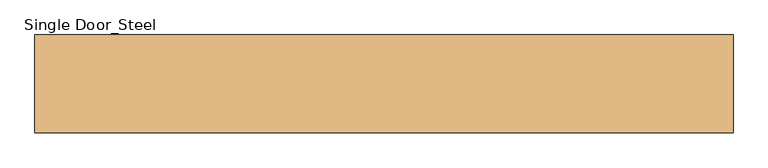
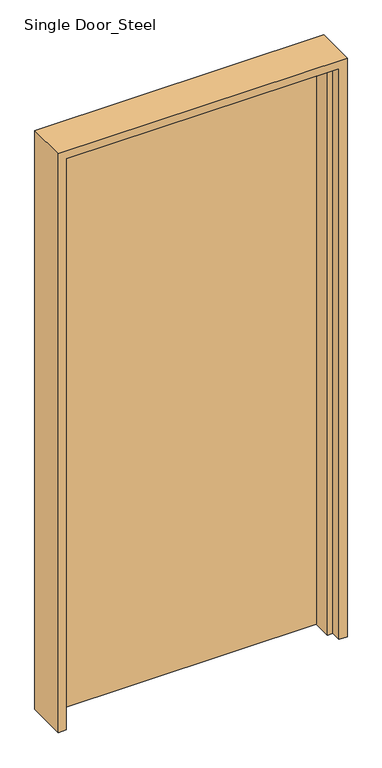
"""IFC4 building model written with IfcOpenShell, lengths in millimetres: door geometry, Single Door_Steel : H_DR_AR B12_Door_Single_W1100xH2280_FR 1.0H_FSD-1."""

from ifc_helpers import new_model, si_unit, origin, origin_with_axes, place, context, project, spatial, polyline, outline, extrude, faceted_brep, source, transform, mapped, element, save


def single_door_steel_2a7c0b4f(model_context):
    return source(origin(), model_context, "Body", "SolidModel", [
        extrude(outline(polyline([(505.0, 75.0), (505.0, 35.0), (-505.0, 35.0), (-505.0, 75.0), (505.0, 75.0)])), origin_with_axes(), (0.0, 0.0, 1.0), 2235.0),
        faceted_brep([(505.0, 75.0, 0.0), (535.0, 75.0, 0.0), (535.0, -75.0, 0.0), (505.0, -75.0, 0.0), (505.0, -35.0, 0.0), (485.0, -35.0, 0.0), (485.0, 35.0, 0.0), (505.0, 35.0, 0.0), (-505.0, 75.0, 0.0), (-505.0, 35.0, 0.0), (-485.0, 35.0, 0.0), (-485.0, -35.0, 0.0), (-505.0, -35.0, 0.0), (-505.0, -75.0, 0.0), (-535.0, -75.0, 0.0), (-535.0, 75.0, 0.0), (505.0, 75.0, 2235.0), (-505.0, 75.0, 2235.0), (-535.0, 75.0, 2265.0), (535.0, 75.0, 2265.0), (535.0, -75.0, 2265.0), (-535.0, -75.0, 2265.0), (-505.0, -75.0, 2235.0), (505.0, -75.0, 2235.0), (505.0, -35.0, 2235.0), (-505.0, -35.0, 2235.0), (-485.0, -35.0, 2215.0), (485.0, -35.0, 2215.0), (485.0, 35.0, 2215.0), (-485.0, 35.0, 2215.0), (-505.0, 35.0, 2235.0), (505.0, 35.0, 2235.0)], [[[0, 1, 2, 3, 4, 5, 6, 7]], [[8, 9, 10, 11, 12, 13, 14, 15]], [[1, 0, 16, 17, 8, 15, 18, 19]], [[2, 1, 19, 20]], [[3, 2, 20, 21, 14, 13, 22, 23]], [[4, 3, 23, 24]], [[5, 4, 24, 25, 12, 11, 26, 27]], [[6, 5, 27, 28]], [[7, 6, 28, 29, 10, 9, 30, 31]], [[0, 7, 31, 16]], [[17, 30, 9, 8]], [[21, 18, 15, 14]], [[25, 22, 13, 12]], [[29, 26, 11, 10]], [[20, 19, 18, 21]], [[24, 23, 22, 25]], [[28, 27, 26, 29]], [[16, 31, 30, 17]]]),
    ])


if __name__ == "__main__":
    model = new_model("IFC4")
    model_context = context("Model", 3, world=origin())
    ifc_project = project(units=[si_unit("LENGTHUNIT", "METRE", prefix="MILLI")], contexts=[model_context])
    site = spatial("IfcSite", under=ifc_project)
    building = spatial("IfcBuilding", under=site)
    placement = place(None, origin())
    single_door_steel_shape = single_door_steel_2a7c0b4f(model_context)
    element("IfcDoor", 1, ObjectType="Single Door_Steel : H_DR_AR B12_Door_Single_W1100xH2280_FR 1.0H_FSD-1", at=placement, inside=building, context=model_context, shape_type="MappedRepresentation", body=[
        mapped(single_door_steel_shape, transform((0.0, 0.0, 0.0), x_axis=(1.0, 0.0, 0.0), y_axis=(0.0, 1.0, 0.0), z_axis=(0.0, 0.0, 1.0))),
    ])
    save(model, "model.ifc")

# Revit data of these elements
# Type "Single Door_Steel : H_DR_AR B12_Door_Single_W1100xH2280_FR 1.0H_FSD-1"
#   Type Mark = "441"
#   Analytic Construction = "<None>"
#   프레임 투영 외부. = 25 mm
#   프레임 투영 내부. = 25 mm
#   프레임 폭 = 75 mm
#   Height = 2280 mm
#   Width = 1100 mm
#   Define Thermal Properties by = 1
#   문 패널 = none
#   문 프레임 = none
#   Function = (empty or 0)
#   Wall Closure = (empty or 0)
